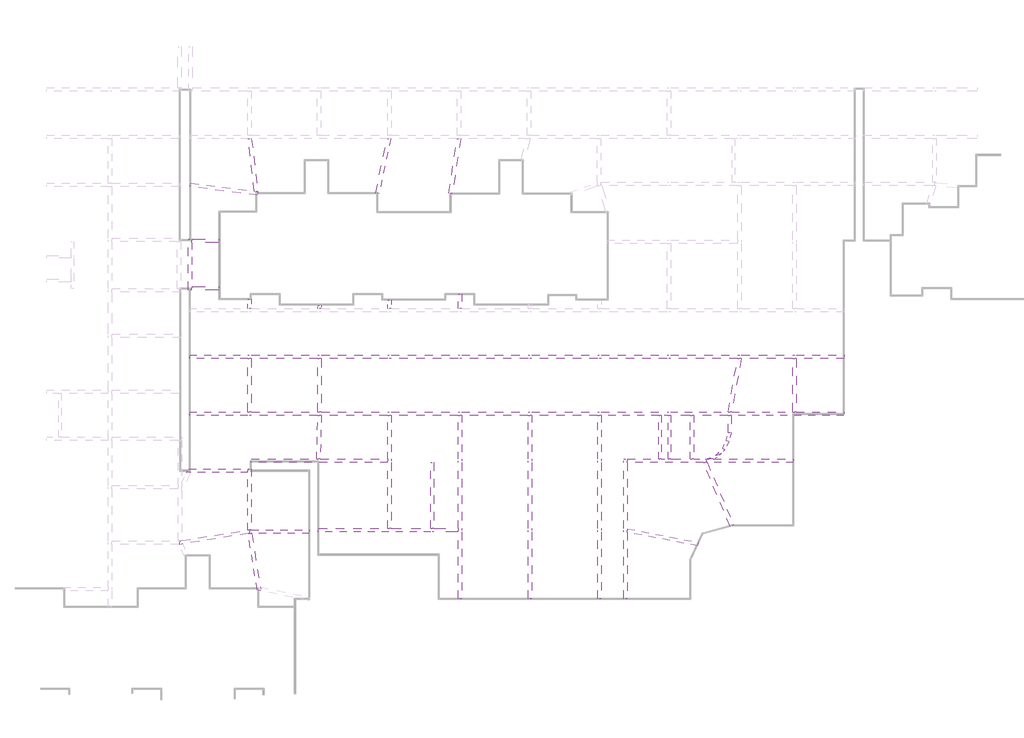
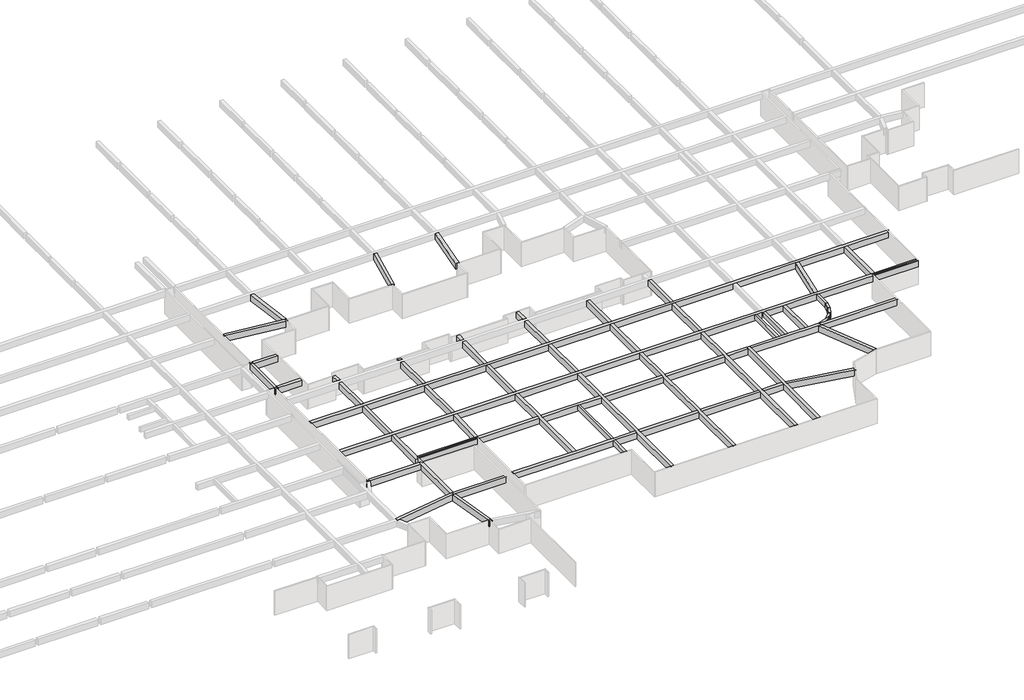
# One storey, part 12 of 16: 43 beams.
"""IFC4 building model written with IfcOpenShell, lengths in millimetres."""

from ifc_helpers import new_model, si_unit, frame, origin, place, context, project, spatial, polyline, outline, extrude, faceted_brep, element, save

model = new_model("IFC4")

# Units and contexts
model_context = context("Model", 3, world=origin())
ifc_project = project(units=[si_unit("LENGTHUNIT", "METRE", prefix="MILLI")], contexts=[model_context])

# Site, building, storey
site = spatial("IfcSite", under=ifc_project)
building = spatial("IfcBuilding", under=site)
storey = spatial("IfcBuildingStorey", under=building, Name="户型图", Elevation=0.0)

# Beams
placement = place(None, origin())
element("IfcBeam", 1, ObjectType="混凝土 - 矩形梁 : KL_beam", at=placement, inside=storey, context=model_context, shape_type="Brep", body=[
    faceted_brep([(256371.9419701, -178694.9170291, 3300.0), (255971.9419701, -178694.9170291, 3300.0), (255971.9419701, -184532.1273283, 3300.0), (256371.9419701, -184532.1273283, 3300.0), (256371.9419701, -184132.1273283, 3300.0), (256371.9419701, -179094.9170291, 3300.0), (256371.9419701, -178694.9170291, 2500.0), (256371.9419701, -184532.1273283, 2500.0), (256371.9419701, -184132.1273283, 2500.0), (256371.9419701, -179094.9170291, 2500.0), (255971.9419701, -178694.9170291, 2500.0), (255971.9419701, -184532.1273283, 2500.0)], [[[0, 1, 2, 3, 4, 5]], [[6, 0, 5, 4, 3, 7, 8, 9]], [[10, 6, 9, 8, 7, 11]], [[1, 10, 11, 2]], [[1, 0, 6, 10]], [[3, 2, 11, 7]]]),
])
element("IfcBeam", 2, ObjectType="混凝土 - 矩形梁 : KL_beam", at=placement, inside=storey, context=model_context, shape_type="Brep", body=[
    faceted_brep([(256229.1427512, -172325.6293063, 3300.0), (256229.1427512, -172325.6293063, 2500.0), (256178.5242086, -172722.4135842, 2500.0), (256178.5242086, -172722.4135842, 3300.0), (263858.3414133, -173702.1428111, 3300.0), (263908.9599559, -173305.3585333, 3300.0), (263499.8534109, -173253.1680152, 3300.0), (263858.3414133, -173702.1428111, 2500.0), (263908.9599559, -173305.3585333, 2500.0), (263499.8534109, -173253.1680152, 2500.0)], [[[0, 1, 2, 3]], [[4, 5, 6, 0, 3]], [[7, 4, 3, 2]], [[8, 7, 2, 1, 9]], [[5, 8, 9, 1, 0, 6]], [[5, 4, 7, 8]]]),
])
element("IfcBeam", 3, ObjectType="混凝土 - 矩形梁 : KL_beam", at=placement, inside=storey, context=model_context, shape_type="SweptSolid", body=[
    extrude(outline(polyline([(259423.0877072, -178694.9170291), (259423.0877072, -179094.9170291), (256371.9419701, -179094.9170291), (256371.9419701, -178694.9170291), (259423.0877072, -178694.9170291)])), frame((0.0, 0.0, 2500.0), z_axis=(0.0, 0.0, 1.0), x_axis=(1.0, 0.0, 0.0)), (0.0, 0.0, 1.0), 800.0),
])
element("IfcBeam", 4, ObjectType="混凝土 - 矩形梁 : KL_beam", at=placement, inside=storey, context=model_context, shape_type="SweptSolid", body=[
    extrude(outline(polyline([(259417.188018, -184132.1273283), (259417.188018, -184532.1273283), (256371.9419701, -184532.1273283), (256371.9419701, -184132.1273283), (259417.188018, -184132.1273283)])), frame((0.0, 0.0, 2500.0), z_axis=(0.0, 0.0, 1.0), x_axis=(1.0, 0.0, 0.0)), (0.0, 0.0, 1.0), 800.0),
])
element("IfcBeam", 5, ObjectType="混凝土 - 矩形梁 : KL_beam", at=placement, inside=storey, context=model_context, shape_type="Brep", body=[
    faceted_brep([(330953.597965, -191962.1668684, 3300.0), (330953.597965, -192362.1668684, 3300.0), (330953.597965, -192362.1668684, 2500.0), (330953.597965, -191962.1668684, 2500.0), (256118.597965, -191962.1668684, 3300.0), (256118.597965, -191962.1668684, 2500.0), (256118.597965, -192362.1668684, 2500.0), (256118.597965, -192362.1668684, 3300.0), (325452.9173169, -191962.1668684, 3300.0), (325052.9173169, -191962.1668684, 3300.0), (319175.2880408, -191962.1668684, 3300.0), (318775.2880408, -191962.1668684, 3300.0), (311075.2880408, -191962.1668684, 3300.0), (310675.2880408, -191962.1668684, 3300.0), (303155.2880408, -191962.1668684, 3300.0), (302755.2880408, -191962.1668684, 3300.0), (295188.9093069, -191962.1668684, 3300.0), (294788.9093069, -191962.1668684, 3300.0), (287188.9093069, -191962.1668684, 3300.0), (286788.9093069, -191962.1668684, 3300.0), (279139.4840766, -191962.1668684, 3300.0), (278739.4840766, -191962.1668684, 3300.0), (271154.6470805, -191962.1668684, 3300.0), (270754.6470805, -191962.1668684, 3300.0), (263153.757676, -191962.1668684, 3300.0), (262753.757676, -191962.1668684, 3300.0), (262753.757676, -192362.1668684, 3300.0), (263153.757676, -192362.1668684, 3300.0), (270754.6470805, -192362.1668684, 3300.0), (271154.6470805, -192362.1668684, 3300.0), (278739.4840766, -192362.1668684, 3300.0), (279139.4840766, -192362.1668684, 3300.0), (286788.9093069, -192362.1668684, 3300.0), (287188.9093069, -192362.1668684, 3300.0), (294788.9093069, -192362.1668684, 3300.0), (295188.9093069, -192362.1668684, 3300.0), (302755.2880408, -192362.1668684, 3300.0), (303155.2880408, -192362.1668684, 3300.0), (310675.2880408, -192362.1668684, 3300.0), (311075.2880408, -192362.1668684, 3300.0), (318737.3738799, -192362.1668684, 3300.0), (319143.4159061, -192362.1668684, 3300.0), (325052.9173169, -192362.1668684, 3300.0), (325452.9173169, -192362.1668684, 3300.0), (262753.757676, -192362.1668684, 2500.0), (263153.757676, -192362.1668684, 2500.0), (270754.6470805, -192362.1668684, 2500.0), (271154.6470805, -192362.1668684, 2500.0), (278739.4840766, -192362.1668684, 2500.0), (279139.4840766, -192362.1668684, 2500.0), (286788.9093069, -192362.1668684, 2500.0), (287188.9093069, -192362.1668684, 2500.0), (294788.9093069, -192362.1668684, 2500.0), (295188.9093069, -192362.1668684, 2500.0), (302755.2880408, -192362.1668684, 2500.0), (303155.2880408, -192362.1668684, 2500.0), (310675.2880408, -192362.1668684, 2500.0), (311075.2880408, -192362.1668684, 2500.0), (318737.3738799, -192362.1668684, 2500.0), (319143.4159061, -192362.1668684, 2500.0), (325052.9173169, -192362.1668684, 2500.0), (325452.9173169, -192362.1668684, 2500.0), (262753.757676, -191962.1668684, 2500.0), (263153.757676, -191962.1668684, 2500.0), (270754.6470805, -191962.1668684, 2500.0), (271154.6470805, -191962.1668684, 2500.0), (278739.4840766, -191962.1668684, 2500.0), (279139.4840766, -191962.1668684, 2500.0), (286788.9093069, -191962.1668684, 2500.0), (287188.9093069, -191962.1668684, 2500.0), (294788.9093069, -191962.1668684, 2500.0), (295188.9093069, -191962.1668684, 2500.0), (302755.2880408, -191962.1668684, 2500.0), (303155.2880408, -191962.1668684, 2500.0), (310675.2880408, -191962.1668684, 2500.0), (311075.2880408, -191962.1668684, 2500.0), (318775.2880408, -191962.1668684, 2500.0), (319175.2880408, -191962.1668684, 2500.0), (325052.9173169, -191962.1668684, 2500.0), (325452.9173169, -191962.1668684, 2500.0)], [[[0, 1, 2, 3]], [[4, 5, 6, 7]], [[1, 0, 8, 9, 10, 11, 12, 13, 14, 15, 16, 17, 18, 19, 20, 21, 22, 23, 24, 25, 4, 7, 26, 27, 28, 29, 30, 31, 32, 33, 34, 35, 36, 37, 38, 39, 40, 41, 42, 43]], [[2, 1, 43, 42, 41, 40, 39, 38, 37, 36, 35, 34, 33, 32, 31, 30, 29, 28, 27, 26, 7, 6, 44, 45, 46, 47, 48, 49, 50, 51, 52, 53, 54, 55, 56, 57, 58, 59, 60, 61]], [[3, 2, 61, 60, 59, 58, 57, 56, 55, 54, 53, 52, 51, 50, 49, 48, 47, 46, 45, 44, 6, 5, 62, 63, 64, 65, 66, 67, 68, 69, 70, 71, 72, 73, 74, 75, 76, 77, 78, 79]], [[0, 3, 79, 78, 77, 76, 75, 74, 73, 72, 71, 70, 69, 68, 67, 66, 65, 64, 63, 62, 5, 4, 25, 24, 23, 22, 21, 20, 19, 18, 17, 16, 15, 14, 13, 12, 11, 10, 9, 8]]]),
])
element("IfcBeam", 6, ObjectType="混凝土 - 矩形梁 : KL_beam", at=placement, inside=storey, context=model_context, shape_type="Brep", body=[
    faceted_brep([(330853.597965, -198470.1471774, 3300.0), (330853.597965, -198870.1471774, 3300.0), (330853.597965, -198870.1471774, 2500.0), (330853.597965, -198470.1471774, 2500.0), (256118.597965, -198470.1471774, 3300.0), (256118.597965, -198470.1471774, 2500.0), (256118.597965, -198870.1471774, 2500.0), (256118.597965, -198870.1471774, 3300.0), (325452.9173169, -198470.1471774, 3300.0), (325052.9173169, -198470.1471774, 3300.0), (318077.7826069, -198470.1471774, 3300.0), (317671.7405807, -198470.1471774, 3300.0), (311075.2880408, -198470.1471774, 3300.0), (310675.2880408, -198470.1471774, 3300.0), (303155.2880408, -198470.1471774, 3300.0), (302755.2880408, -198470.1471774, 3300.0), (295188.9093069, -198470.1471774, 3300.0), (294788.9093069, -198470.1471774, 3300.0), (287188.9093069, -198470.1471774, 3300.0), (286788.9093069, -198470.1471774, 3300.0), (279139.4840766, -198470.1471774, 3300.0), (278739.4840766, -198470.1471774, 3300.0), (271154.6470805, -198470.1471774, 3300.0), (270754.6470805, -198470.1471774, 3300.0), (263153.757676, -198470.1471774, 3300.0), (262753.757676, -198470.1471774, 3300.0), (262753.757676, -198870.1471774, 3300.0), (263153.757676, -198870.1471774, 3300.0), (270749.982593, -198870.1471774, 3300.0), (271150.0889009, -198870.1471774, 3300.0), (278739.4840766, -198870.1471774, 3300.0), (279139.4840766, -198870.1471774, 3300.0), (286788.9093069, -198870.1471774, 3300.0), (287188.9093069, -198870.1471774, 3300.0), (294788.9093069, -198870.1471774, 3300.0), (295188.9093069, -198870.1471774, 3300.0), (302755.2880408, -198870.1471774, 3300.0), (303155.2880408, -198870.1471774, 3300.0), (309705.2880408, -198870.1471774, 3300.0), (310005.2880408, -198870.1471774, 3300.0), (310675.2880408, -198870.1471774, 3300.0), (310805.2880408, -198870.1471774, 3300.0), (311105.2880408, -198870.1471774, 3300.0), (313355.2880408, -198870.1471774, 3300.0), (313755.2880408, -198870.1471774, 3300.0), (317689.868446, -198870.1471774, 3300.0), (317989.868446, -198870.1471774, 3300.0), (262753.757676, -198870.1471774, 2500.0), (263153.757676, -198870.1471774, 2500.0), (270749.982593, -198870.1471774, 2500.0), (271150.0889009, -198870.1471774, 2500.0), (278739.4840766, -198870.1471774, 2500.0), (279139.4840766, -198870.1471774, 2500.0), (286788.9093069, -198870.1471774, 2500.0), (287188.9093069, -198870.1471774, 2500.0), (294788.9093069, -198870.1471774, 2500.0), (295188.9093069, -198870.1471774, 2500.0), (302755.2880408, -198870.1471774, 2500.0), (303155.2880408, -198870.1471774, 2500.0), (310675.2880408, -198870.1471774, 2500.0), (311075.2880408, -198870.1471774, 2500.0), (313355.2880408, -198870.1471774, 2500.0), (313755.2880408, -198870.1471774, 2500.0), (262753.757676, -198470.1471774, 2500.0), (263153.757676, -198470.1471774, 2500.0), (270754.6470805, -198470.1471774, 2500.0), (271154.6470805, -198470.1471774, 2500.0), (278739.4840766, -198470.1471774, 2500.0), (279139.4840766, -198470.1471774, 2500.0), (286788.9093069, -198470.1471774, 2500.0), (287188.9093069, -198470.1471774, 2500.0), (294788.9093069, -198470.1471774, 2500.0), (295188.9093069, -198470.1471774, 2500.0), (302755.2880408, -198470.1471774, 2500.0), (303155.2880408, -198470.1471774, 2500.0), (310675.2880408, -198470.1471774, 2500.0), (311075.2880408, -198470.1471774, 2500.0), (317671.7405807, -198470.1471774, 2500.0), (318077.7826069, -198470.1471774, 2500.0), (325052.9173169, -198470.1471774, 2500.0), (325452.9173169, -198470.1471774, 2500.0)], [[[0, 1, 2, 3]], [[4, 5, 6, 7]], [[1, 0, 8, 9, 10, 11, 12, 13, 14, 15, 16, 17, 18, 19, 20, 21, 22, 23, 24, 25, 4, 7, 26, 27, 28, 29, 30, 31, 32, 33, 34, 35, 36, 37, 38, 39, 40, 41, 42, 43, 44, 45, 46]], [[2, 1, 46, 45, 44, 43, 42, 41, 40, 39, 38, 37, 36, 35, 34, 33, 32, 31, 30, 29, 28, 27, 26, 7, 6, 47, 48, 49, 50, 51, 52, 53, 54, 55, 56, 57, 58, 59, 60, 61, 62]], [[3, 2, 62, 61, 60, 59, 58, 57, 56, 55, 54, 53, 52, 51, 50, 49, 48, 47, 6, 5, 63, 64, 65, 66, 67, 68, 69, 70, 71, 72, 73, 74, 75, 76, 77, 78, 79, 80]], [[0, 3, 80, 79, 78, 77, 76, 75, 74, 73, 72, 71, 70, 69, 68, 67, 66, 65, 64, 63, 5, 4, 25, 24, 23, 22, 21, 20, 19, 18, 17, 16, 15, 14, 13, 12, 11, 10, 9, 8]]]),
])
element("IfcBeam", 7, ObjectType="混凝土 - 矩形梁 : KL_beam", at=placement, inside=storey, context=model_context, shape_type="Brep", body=[
    faceted_brep([(262753.757676, -204304.6570229, 3300.0), (262753.757676, -204304.6570229, 2500.0), (263153.757676, -204304.6570229, 2500.0), (263153.757676, -204304.6570229, 3300.0), (262753.757676, -198870.1471774, 3300.0), (263153.757676, -198870.1471774, 3300.0), (263153.757676, -198870.1471774, 2500.0), (262753.757676, -198870.1471774, 2500.0), (263153.757676, -204273.7545432, 3300.0), (263153.757676, -203873.7545432, 3300.0), (263153.757676, -204273.7545432, 2500.0), (263153.757676, -203873.7545432, 2500.0)], [[[0, 1, 2, 3]], [[4, 5, 6, 7]], [[0, 3, 8, 9, 5, 4]], [[3, 2, 10, 11, 6, 5, 9, 8]], [[2, 1, 7, 6, 11, 10]], [[1, 0, 4, 7]]]),
    faceted_brep([(263153.757676, -187062.1668684, 3300.0), (262753.757676, -187062.1668684, 3300.0), (262753.757676, -191962.1668684, 3300.0), (263153.757676, -191962.1668684, 3300.0), (263153.757676, -187062.1668684, 2500.0), (263153.757676, -191962.1668684, 2500.0), (262753.757676, -187062.1668684, 2500.0), (262753.757676, -191962.1668684, 2500.0)], [[[0, 1, 2, 3]], [[4, 0, 3, 5]], [[6, 4, 5, 7]], [[1, 6, 7, 2]], [[1, 0, 4, 6]], [[3, 2, 7, 5]]]),
    faceted_brep([(262753.757676, -192362.1668684, 3300.0), (263153.757676, -192362.1668684, 3300.0), (263153.757676, -192362.1668684, 2500.0), (262753.757676, -192362.1668684, 2500.0), (262753.757676, -198470.1471774, 3300.0), (263153.757676, -198470.1471774, 3300.0), (263153.757676, -198470.1471774, 2500.0), (262753.757676, -198470.1471774, 2500.0)], [[[0, 1, 2, 3]], [[1, 0, 4, 5]], [[2, 1, 5, 6]], [[3, 2, 6, 7]], [[0, 3, 7, 4]], [[5, 4, 7, 6]]]),
])
element("IfcBeam", 8, ObjectType="混凝土 - 矩形梁 : KL_beam", at=placement, inside=storey, context=model_context, shape_type="SweptSolid", body=[
    extrude(outline(polyline([(270754.6470805, -187062.1668684), (271154.6470805, -187062.1668684), (271154.6470805, -191962.1668684), (270754.6470805, -191962.1668684), (270754.6470805, -187062.1668684)])), frame((0.0, 0.0, 2500.0), z_axis=(0.0, 0.0, 1.0), x_axis=(1.0, 0.0, 0.0)), (0.0, 0.0, 1.0), 800.0),
    extrude(outline(polyline([(271154.6470805, -198470.1471774), (270754.6470805, -198470.1471774), (270754.6470805, -192362.1668684), (271154.6470805, -192362.1668684), (271154.6470805, -198470.1471774)])), frame((0.0, 0.0, 2500.0), z_axis=(0.0, 0.0, 1.0), x_axis=(1.0, 0.0, 0.0)), (0.0, 0.0, 1.0), 800.0),
])
element("IfcBeam", 9, ObjectType="混凝土 - 矩形梁 : KL_beam", at=placement, inside=storey, context=model_context, shape_type="SweptSolid", body=[
    extrude(outline(polyline([(270749.982593, -198870.1471774), (271150.0889009, -198870.1471774), (271034.7223897, -203873.7545432), (270634.6160818, -203873.7545432), (270749.982593, -198870.1471774)])), frame((0.0, 0.0, 2500.0), z_axis=(0.0, 0.0, 1.0), x_axis=(1.0, 0.0, 0.0)), (0.0, 0.0, 1.0), 800.0),
])
element("IfcBeam", 10, ObjectType="混凝土 - 矩形梁 : KL_beam", at=placement, inside=storey, context=model_context, shape_type="Brep", body=[
    faceted_brep([(279139.4840766, -198870.1471774, 3300.0), (278739.4840766, -198870.1471774, 3300.0), (278739.4840766, -203873.7545432, 3300.0), (278739.4840766, -204273.7545432, 3300.0), (278739.4840766, -211805.8350287, 3300.0), (279139.4840766, -211805.8350287, 3300.0), (279139.4840766, -204273.7545432, 3300.0), (279139.4840766, -203873.7545432, 3300.0), (279139.4840766, -198870.1471774, 2500.0), (279139.4840766, -211805.8350287, 2500.0), (279139.4840766, -204273.7545432, 2500.0), (279139.4840766, -203873.7545432, 2500.0), (278739.4840766, -198870.1471774, 2500.0), (278739.4840766, -211805.8350287, 2500.0), (278739.4840766, -204273.7545432, 2500.0), (278739.4840766, -203873.7545432, 2500.0)], [[[0, 1, 2, 3, 4, 5, 6, 7]], [[8, 0, 7, 6, 5, 9, 10, 11]], [[12, 8, 11, 10, 9, 13, 14, 15]], [[1, 12, 15, 14, 13, 4, 3, 2]], [[1, 0, 8, 12]], [[5, 4, 13, 9]]]),
    faceted_brep([(278739.4840766, -187062.1668684, 3300.0), (279139.4840766, -187062.1668684, 3300.0), (279139.4840766, -187062.1668684, 2500.0), (278739.4840766, -187062.1668684, 2500.0), (279139.4840766, -191962.1668684, 3300.0), (278739.4840766, -191962.1668684, 3300.0), (278739.4840766, -191962.1668684, 2500.0), (279139.4840766, -191962.1668684, 2500.0)], [[[0, 1, 2, 3]], [[4, 5, 6, 7]], [[1, 0, 5, 4]], [[2, 1, 4, 7]], [[3, 2, 7, 6]], [[0, 3, 6, 5]]]),
    faceted_brep([(278739.4840766, -192362.1668684, 3300.0), (279139.4840766, -192362.1668684, 3300.0), (279139.4840766, -192362.1668684, 2500.0), (278739.4840766, -192362.1668684, 2500.0), (279139.4840766, -198470.1471774, 3300.0), (278739.4840766, -198470.1471774, 3300.0), (278739.4840766, -198470.1471774, 2500.0), (279139.4840766, -198470.1471774, 2500.0)], [[[0, 1, 2, 3]], [[4, 5, 6, 7]], [[1, 0, 5, 4]], [[2, 1, 4, 7]], [[3, 2, 7, 6]], [[0, 3, 6, 5]]]),
])
element("IfcBeam", 11, ObjectType="混凝土 - 矩形梁 : KL_beam", at=placement, inside=storey, context=model_context, shape_type="Brep", body=[
    faceted_brep([(287188.9093069, -219873.4607058, 3300.0), (286788.9093069, -219873.4607058, 3300.0), (286788.9093069, -219873.4607058, 2500.0), (287188.9093069, -219873.4607058, 2500.0), (287188.9093069, -212205.8350287, 3300.0), (287188.9093069, -211805.8350287, 3300.0), (287188.9093069, -204273.7545432, 3300.0), (287188.9093069, -203873.7545432, 3300.0), (287188.9093069, -198870.1471774, 3300.0), (286788.9093069, -198870.1471774, 3300.0), (286788.9093069, -203873.7545432, 3300.0), (286788.9093069, -204273.7545432, 3300.0), (286788.9093069, -211805.8350287, 3300.0), (286788.9093069, -212205.8350287, 3300.0), (286788.9093069, -198870.1471774, 2500.0), (286788.9093069, -203873.7545432, 2500.0), (286788.9093069, -204273.7545432, 2500.0), (286788.9093069, -211805.8350287, 2500.0), (286788.9093069, -212205.8350287, 2500.0), (287188.9093069, -198870.1471774, 2500.0), (287188.9093069, -203873.7545432, 2500.0), (287188.9093069, -204273.7545432, 2500.0), (287188.9093069, -211805.8350287, 2500.0), (287188.9093069, -212205.8350287, 2500.0)], [[[0, 1, 2, 3]], [[1, 0, 4, 5, 6, 7, 8, 9, 10, 11, 12, 13]], [[2, 1, 13, 12, 11, 10, 9, 14, 15, 16, 17, 18]], [[3, 2, 18, 17, 16, 15, 14, 19, 20, 21, 22, 23]], [[0, 3, 23, 22, 21, 20, 19, 8, 7, 6, 5, 4]], [[9, 8, 19, 14]]]),
    faceted_brep([(286788.9093069, -187062.1668684, 3300.0), (287188.9093069, -187062.1668684, 3300.0), (287188.9093069, -187062.1668684, 2500.0), (286788.9093069, -187062.1668684, 2500.0), (287188.9093069, -191962.1668684, 3300.0), (286788.9093069, -191962.1668684, 3300.0), (286788.9093069, -191962.1668684, 2500.0), (287188.9093069, -191962.1668684, 2500.0)], [[[0, 1, 2, 3]], [[4, 5, 6, 7]], [[1, 0, 5, 4]], [[0, 3, 6, 5]], [[3, 2, 7, 6]], [[2, 1, 4, 7]]]),
    faceted_brep([(286788.9093069, -192362.1668684, 3300.0), (287188.9093069, -192362.1668684, 3300.0), (287188.9093069, -192362.1668684, 2500.0), (286788.9093069, -192362.1668684, 2500.0), (287188.9093069, -198470.1471774, 3300.0), (286788.9093069, -198470.1471774, 3300.0), (286788.9093069, -198470.1471774, 2500.0), (287188.9093069, -198470.1471774, 2500.0)], [[[0, 1, 2, 3]], [[4, 5, 6, 7]], [[1, 0, 5, 4]], [[0, 3, 6, 5]], [[3, 2, 7, 6]], [[2, 1, 4, 7]]]),
])
element("IfcBeam", 12, ObjectType="混凝土 - 矩形梁 : KL_beam", at=placement, inside=storey, context=model_context, shape_type="Brep", body=[
    faceted_brep([(294788.9093069, -219873.4607058, 3300.0), (294788.9093069, -219873.4607058, 2500.0), (295188.9093069, -219873.4607058, 2500.0), (295188.9093069, -219873.4607058, 3300.0), (294788.9093069, -198870.1471774, 3300.0), (295188.9093069, -198870.1471774, 3300.0), (295188.9093069, -198870.1471774, 2500.0), (294788.9093069, -198870.1471774, 2500.0), (295188.9093069, -212205.8350287, 3300.0), (295188.9093069, -211805.8350287, 3300.0), (295188.9093069, -204273.7545432, 3300.0), (295188.9093069, -203873.7545432, 3300.0), (294788.9093069, -203873.7545432, 3300.0), (294788.9093069, -204273.7545432, 3300.0), (294788.9093069, -211805.8350287, 3300.0), (294788.9093069, -212205.8350287, 3300.0), (295188.9093069, -212205.8350287, 2500.0), (295188.9093069, -211805.8350287, 2500.0), (295188.9093069, -204273.7545432, 2500.0), (295188.9093069, -203873.7545432, 2500.0), (294788.9093069, -212205.8350287, 2500.0), (294788.9093069, -211805.8350287, 2500.0), (294788.9093069, -204273.7545432, 2500.0), (294788.9093069, -203873.7545432, 2500.0)], [[[0, 1, 2, 3]], [[4, 5, 6, 7]], [[0, 3, 8, 9, 10, 11, 5, 4, 12, 13, 14, 15]], [[3, 2, 16, 17, 18, 19, 6, 5, 11, 10, 9, 8]], [[2, 1, 20, 21, 22, 23, 7, 6, 19, 18, 17, 16]], [[1, 0, 15, 14, 13, 12, 4, 7, 23, 22, 21, 20]]]),
    faceted_brep([(295188.9093069, -187062.1668684, 3300.0), (294788.9093069, -187062.1668684, 3300.0), (294788.9093069, -191962.1668684, 3300.0), (295188.9093069, -191962.1668684, 3300.0), (295188.9093069, -187062.1668684, 2500.0), (295188.9093069, -191962.1668684, 2500.0), (294788.9093069, -187062.1668684, 2500.0), (294788.9093069, -191962.1668684, 2500.0)], [[[0, 1, 2, 3]], [[4, 0, 3, 5]], [[6, 4, 5, 7]], [[1, 6, 7, 2]], [[1, 0, 4, 6]], [[3, 2, 7, 5]]]),
    faceted_brep([(294788.9093069, -192362.1668684, 3300.0), (295188.9093069, -192362.1668684, 3300.0), (295188.9093069, -192362.1668684, 2500.0), (294788.9093069, -192362.1668684, 2500.0), (294788.9093069, -198470.1471774, 3300.0), (295188.9093069, -198470.1471774, 3300.0), (295188.9093069, -198470.1471774, 2500.0), (294788.9093069, -198470.1471774, 2500.0)], [[[0, 1, 2, 3]], [[1, 0, 4, 5]], [[2, 1, 5, 6]], [[3, 2, 6, 7]], [[0, 3, 7, 4]], [[5, 4, 7, 6]]]),
])
element("IfcBeam", 13, ObjectType="混凝土 - 矩形梁 : KL_beam", at=placement, inside=storey, context=model_context, shape_type="Brep", body=[
    faceted_brep([(303155.2880408, -219873.4607058, 3300.0), (302755.2880408, -219873.4607058, 3300.0), (302755.2880408, -219873.4607058, 2500.0), (303155.2880408, -219873.4607058, 2500.0), (303155.2880408, -212205.8350287, 3300.0), (303155.2880408, -211805.8350287, 3300.0), (303155.2880408, -204273.7545432, 3300.0), (303155.2880408, -203873.7545432, 3300.0), (303155.2880408, -198870.1471774, 3300.0), (302755.2880408, -198870.1471774, 3300.0), (302755.2880408, -203873.7545432, 3300.0), (302755.2880408, -204273.7545432, 3300.0), (302755.2880408, -211805.8350287, 3300.0), (302755.2880408, -212205.8350287, 3300.0), (302755.2880408, -198870.1471774, 2500.0), (302755.2880408, -203873.7545432, 2500.0), (302755.2880408, -204273.7545432, 2500.0), (302755.2880408, -211805.8350287, 2500.0), (302755.2880408, -212205.8350287, 2500.0), (303155.2880408, -198870.1471774, 2500.0), (303155.2880408, -203873.7545432, 2500.0), (303155.2880408, -204273.7545432, 2500.0), (303155.2880408, -211805.8350287, 2500.0), (303155.2880408, -212205.8350287, 2500.0)], [[[0, 1, 2, 3]], [[1, 0, 4, 5, 6, 7, 8, 9, 10, 11, 12, 13]], [[2, 1, 13, 12, 11, 10, 9, 14, 15, 16, 17, 18]], [[3, 2, 18, 17, 16, 15, 14, 19, 20, 21, 22, 23]], [[0, 3, 23, 22, 21, 20, 19, 8, 7, 6, 5, 4]], [[9, 8, 19, 14]]]),
    faceted_brep([(302755.2880408, -187062.1668684, 3300.0), (303155.2880408, -187062.1668684, 3300.0), (303155.2880408, -187062.1668684, 2500.0), (302755.2880408, -187062.1668684, 2500.0), (303155.2880408, -191962.1668684, 3300.0), (302755.2880408, -191962.1668684, 3300.0), (302755.2880408, -191962.1668684, 2500.0), (303155.2880408, -191962.1668684, 2500.0)], [[[0, 1, 2, 3]], [[4, 5, 6, 7]], [[1, 0, 5, 4]], [[0, 3, 6, 5]], [[3, 2, 7, 6]], [[2, 1, 4, 7]]]),
    faceted_brep([(302755.2880408, -192362.1668684, 3300.0), (303155.2880408, -192362.1668684, 3300.0), (303155.2880408, -192362.1668684, 2500.0), (302755.2880408, -192362.1668684, 2500.0), (303155.2880408, -198470.1471774, 3300.0), (302755.2880408, -198470.1471774, 3300.0), (302755.2880408, -198470.1471774, 2500.0), (303155.2880408, -198470.1471774, 2500.0)], [[[0, 1, 2, 3]], [[4, 5, 6, 7]], [[1, 0, 5, 4]], [[0, 3, 6, 5]], [[3, 2, 7, 6]], [[2, 1, 4, 7]]]),
])
element("IfcBeam", 14, ObjectType="混凝土 - 矩形梁 : KL_beam", at=placement, inside=storey, context=model_context, shape_type="Brep", body=[
    faceted_brep([(305755.2880408, -219873.7545432, 3300.0), (305755.2880408, -219873.7545432, 2500.0), (306155.2880408, -219873.7545432, 2500.0), (306155.2880408, -219873.7545432, 3300.0), (306155.2880408, -212248.4544295, 3300.0), (306155.2880408, -211840.9677515, 3300.0), (306155.2880408, -204273.7545432, 3300.0), (306155.2880408, -203873.7545432, 3300.0), (305755.2880408, -203873.7545432, 3300.0), (305755.2880408, -204273.7545432, 3300.0), (305755.2880408, -211805.8350287, 3300.0), (305755.2880408, -212205.8350287, 3300.0), (306155.2880408, -212248.4544295, 2500.0), (306155.2880408, -211840.9677515, 2500.0), (306155.2880408, -204273.7545432, 2500.0), (306155.2880408, -203873.7545432, 2500.0), (305755.2880408, -212205.8350287, 2500.0), (305755.2880408, -211805.8350287, 2500.0), (305755.2880408, -204273.7545432, 2500.0), (305755.2880408, -203873.7545432, 2500.0)], [[[0, 1, 2, 3]], [[0, 3, 4, 5, 6, 7, 8, 9, 10, 11]], [[3, 2, 12, 13, 14, 15, 7, 6, 5, 4]], [[2, 1, 16, 17, 18, 19, 15, 14, 13, 12]], [[1, 0, 11, 10, 9, 8, 19, 18, 17, 16]], [[8, 7, 15, 19]]]),
])
element("IfcBeam", 15, ObjectType="混凝土 - 矩形梁 : KL_beam", at=placement, inside=storey, context=model_context, shape_type="Brep", body=[
    faceted_brep([(315257.2223737, -204273.7545432, 3300.0), (315087.7671783, -203873.7545432, 3300.0), (315066.2128647, -203873.7545432, 3300.0), (313755.2880408, -203873.7545432, 3300.0), (313355.2880408, -203873.7545432, 3300.0), (311105.2880408, -203873.7545432, 3300.0), (310805.2880408, -203873.7545432, 3300.0), (310005.2880408, -203873.7545432, 3300.0), (309705.2880408, -203873.7545432, 3300.0), (306155.2880408, -203873.7545432, 3300.0), (306155.2880408, -204273.7545432, 3300.0), (314822.8089033, -204273.7545432, 3300.0), (315257.2223737, -204273.7545432, 2500.0), (306155.2880408, -204273.7545432, 2500.0), (314822.8089033, -204273.7545432, 2500.0), (315087.7671783, -203873.7545432, 2500.0), (306155.2880408, -203873.7545432, 2500.0), (313355.2880408, -203873.7545432, 2500.0), (313755.2880408, -203873.7545432, 2500.0)], [[[0, 1, 2, 3, 4, 5, 6, 7, 8, 9, 10, 11]], [[12, 0, 11, 10, 13, 14]], [[15, 12, 14, 13, 16, 17, 18]], [[1, 15, 18, 17, 16, 9, 8, 7, 6, 5, 4, 3, 2]], [[10, 9, 16, 13]], [[1, 0, 12, 15]]]),
])
element("IfcBeam", 16, ObjectType="混凝土 - 矩形梁 : KL_beam", at=placement, inside=storey, context=model_context, shape_type="Brep", body=[
    faceted_brep([(325092.6026789, -203873.7545432, 3300.0), (325092.6026789, -204273.7545432, 3300.0), (325092.6026789, -204273.7545432, 2500.0), (325092.6026789, -203873.7545432, 2500.0), (315943.3541847, -203873.7545432, 3300.0), (315087.7671783, -203873.7545432, 3300.0), (315257.2223737, -204273.7545432, 3300.0), (315257.2223737, -204273.7545432, 2500.0), (315087.7671783, -203873.7545432, 2500.0)], [[[0, 1, 2, 3]], [[1, 0, 4, 5, 6]], [[2, 1, 6, 7]], [[3, 2, 7, 8]], [[0, 3, 8, 5, 4]], [[6, 5, 8, 7]]]),
])
element("IfcBeam", 17, ObjectType="混凝土 - 矩形梁 : KL_beam", at=placement, inside=storey, context=model_context, shape_type="SweptSolid", body=[
    extrude(outline(polyline([(313355.2880408, -198870.1471774), (313755.2880408, -198870.1471774), (313755.2880408, -203873.7545432), (313355.2880408, -203873.7545432), (313355.2880408, -198870.1471774)])), frame((0.0, 0.0, 2500.0), z_axis=(0.0, 0.0, 1.0), x_axis=(1.0, 0.0, 0.0)), (0.0, 0.0, 1.0), 800.0),
])
element("IfcBeam", 18, ObjectType="混凝土 - 矩形梁 : KL_beam", at=placement, inside=storey, context=model_context, shape_type="Brep", body=[
    faceted_brep([(305755.2880408, -204273.7545432, 3300.0), (305755.2880408, -203873.7545432, 3300.0), (303155.2880408, -203873.7545432, 3300.0), (303155.2880408, -204273.7545432, 3300.0), (305755.2880408, -203873.7545432, 2500.0), (303155.2880408, -203873.7545432, 2500.0), (305755.2880408, -204273.7545432, 2500.0), (303155.2880408, -204273.7545432, 2500.0)], [[[0, 1, 2, 3]], [[1, 4, 5, 2]], [[4, 6, 7, 5]], [[6, 0, 3, 7]], [[1, 0, 6, 4]], [[3, 2, 5, 7]]]),
    faceted_brep([(263153.757676, -204273.7545432, 3300.0), (263153.757676, -203873.7545432, 3300.0), (263153.757676, -203873.7545432, 2500.0), (263153.757676, -204273.7545432, 2500.0), (278739.4840766, -203873.7545432, 3300.0), (278739.4840766, -204273.7545432, 3300.0), (278739.4840766, -204273.7545432, 2500.0), (278739.4840766, -203873.7545432, 2500.0), (271034.7223897, -203873.7545432, 3300.0), (270634.6160818, -203873.7545432, 3300.0), (271034.7223897, -203873.7545432, 2500.0), (270634.6160818, -203873.7545432, 2500.0)], [[[0, 1, 2, 3]], [[4, 5, 6, 7]], [[1, 0, 5, 4, 8, 9]], [[2, 1, 9, 8, 4, 7, 10, 11]], [[3, 2, 11, 10, 7, 6]], [[0, 3, 6, 5]]]),
    faceted_brep([(279139.4840766, -204273.7545432, 3300.0), (279139.4840766, -203873.7545432, 3300.0), (279139.4840766, -203873.7545432, 2500.0), (279139.4840766, -204273.7545432, 2500.0), (286788.9093069, -203873.7545432, 3300.0), (286788.9093069, -204273.7545432, 3300.0), (286788.9093069, -204273.7545432, 2500.0), (286788.9093069, -203873.7545432, 2500.0), (283693.7576761, -204273.7545432, 3300.0), (283993.7576761, -204273.7545432, 3300.0)], [[[0, 1, 2, 3]], [[4, 5, 6, 7]], [[1, 0, 8, 9, 5, 4]], [[2, 1, 4, 7]], [[3, 2, 7, 6]], [[0, 3, 6, 5, 9, 8]]]),
    faceted_brep([(287188.9093069, -204273.7545432, 3300.0), (287188.9093069, -203873.7545432, 3300.0), (287188.9093069, -203873.7545432, 2500.0), (287188.9093069, -204273.7545432, 2500.0), (294788.9093069, -203873.7545432, 3300.0), (294788.9093069, -204273.7545432, 3300.0), (294788.9093069, -204273.7545432, 2500.0), (294788.9093069, -203873.7545432, 2500.0)], [[[0, 1, 2, 3]], [[4, 5, 6, 7]], [[1, 0, 5, 4]], [[2, 1, 4, 7]], [[3, 2, 7, 6]], [[0, 3, 6, 5]]]),
    faceted_brep([(295188.9093069, -204273.7545432, 3300.0), (295188.9093069, -203873.7545432, 3300.0), (295188.9093069, -203873.7545432, 2500.0), (295188.9093069, -204273.7545432, 2500.0), (302755.2880408, -203873.7545432, 3300.0), (302755.2880408, -204273.7545432, 3300.0), (302755.2880408, -204273.7545432, 2500.0), (302755.2880408, -203873.7545432, 2500.0)], [[[0, 1, 2, 3]], [[4, 5, 6, 7]], [[1, 0, 5, 4]], [[2, 1, 4, 7]], [[3, 2, 7, 6]], [[0, 3, 6, 5]]]),
])
element("IfcBeam", 19, ObjectType="混凝土 - 矩形梁 : KL_beam", at=placement, inside=storey, context=model_context, shape_type="Brep", body=[
    faceted_brep([(270829.0228584, -211805.8350287, 3300.0), (270829.0228584, -211805.8350287, 2500.0), (270829.0228584, -212205.8350287, 2500.0), (270829.0228584, -212205.8350287, 3300.0), (286788.9093069, -211805.8350287, 3300.0), (286788.9093069, -212205.8350287, 3300.0), (286788.9093069, -212205.8350287, 2500.0), (286788.9093069, -211805.8350287, 2500.0), (283693.7576761, -212205.8350287, 3300.0), (283993.7576761, -212205.8350287, 3300.0), (283993.7576761, -211805.8350287, 3300.0), (283693.7576761, -211805.8350287, 3300.0), (279139.4840766, -211805.8350287, 3300.0), (278739.4840766, -211805.8350287, 3300.0), (278739.4840766, -211805.8350287, 2500.0), (279139.4840766, -211805.8350287, 2500.0)], [[[0, 1, 2, 3]], [[4, 5, 6, 7]], [[0, 3, 8, 9, 5, 4, 10, 11, 12, 13]], [[3, 2, 6, 5, 9, 8]], [[2, 1, 14, 15, 7, 6]], [[1, 0, 13, 12, 11, 10, 4, 7, 15, 14]]]),
    faceted_brep([(287188.9093069, -211805.8350287, 3300.0), (287188.9093069, -212205.8350287, 3300.0), (294788.9093069, -212205.8350287, 3300.0), (294788.9093069, -211805.8350287, 3300.0), (287188.9093069, -212205.8350287, 2500.0), (294788.9093069, -212205.8350287, 2500.0), (287188.9093069, -211805.8350287, 2500.0), (294788.9093069, -211805.8350287, 2500.0)], [[[0, 1, 2, 3]], [[1, 4, 5, 2]], [[4, 6, 7, 5]], [[6, 0, 3, 7]], [[1, 0, 6, 4]], [[3, 2, 5, 7]]]),
    faceted_brep([(305755.2880408, -211805.8350287, 3300.0), (305755.2880408, -212205.8350287, 3300.0), (305755.2880408, -212205.8350287, 2500.0), (305755.2880408, -211805.8350287, 2500.0), (303155.2880408, -211805.8350287, 3300.0), (303155.2880408, -212205.8350287, 3300.0), (303155.2880408, -212205.8350287, 2500.0), (303155.2880408, -211805.8350287, 2500.0)], [[[0, 1, 2, 3]], [[1, 0, 4, 5]], [[2, 1, 5, 6]], [[3, 2, 6, 7]], [[0, 3, 7, 4]], [[5, 4, 7, 6]]]),
    faceted_brep([(295188.9093069, -212205.8350287, 3300.0), (295188.9093069, -211805.8350287, 3300.0), (295188.9093069, -211805.8350287, 2500.0), (295188.9093069, -212205.8350287, 2500.0), (302755.2880408, -211805.8350287, 3300.0), (302755.2880408, -212205.8350287, 3300.0), (302755.2880408, -212205.8350287, 2500.0), (302755.2880408, -211805.8350287, 2500.0)], [[[0, 1, 2, 3]], [[4, 5, 6, 7]], [[1, 0, 5, 4]], [[0, 3, 6, 5]], [[3, 2, 7, 6]], [[2, 1, 4, 7]]]),
])
element("IfcBeam", 20, ObjectType="混凝土 - 矩形梁 : KL_beam", at=placement, inside=storey, context=model_context, shape_type="SweptSolid", body=[
    extrude(outline(polyline([(314239.1181809, -213412.3051532), (314162.7945827, -213804.9560265), (306155.2880408, -212248.4544295), (306155.2880408, -211840.9677515), (314239.1181809, -213412.3051532)])), frame((0.0, 0.0, 2500.0), z_axis=(0.0, 0.0, 1.0), x_axis=(1.0, 0.0, 0.0)), (0.0, 0.0, 1.0), 800.0),
])
element("IfcBeam", 21, ObjectType="混凝土 - 矩形梁 : KL_beam", at=placement, inside=storey, context=model_context, shape_type="SweptSolid", body=[
    extrude(outline(polyline([(318276.9582415, -211401.8590835), (317908.6455373, -211557.8903366), (314822.8089033, -204273.7545432), (315257.2223737, -204273.7545432), (318276.9582415, -211401.8590835)])), frame((0.0, 0.0, 2500.0), z_axis=(0.0, 0.0, 1.0), x_axis=(1.0, 0.0, 0.0)), (0.0, 0.0, 1.0), 800.0),
])
element("IfcBeam", 22, ObjectType="混凝土 - 矩形梁 : KL_beam", at=placement, inside=storey, context=model_context, shape_type="SweptSolid", body=[
    extrude(outline(polyline([(286788.9093069, -185002.1668684), (287188.9093069, -185002.1668684), (287188.9093069, -186662.1668684), (286788.9093069, -186662.1668684), (286788.9093069, -185002.1668684)])), frame((0.0, 0.0, 2500.0), z_axis=(0.0, 0.0, 1.0), x_axis=(1.0, 0.0, 0.0)), (0.0, 0.0, 1.0), 800.0),
])
element("IfcBeam", 23, ObjectType="混凝土 - 矩形梁 : KL_beam", at=placement, inside=storey, context=model_context, shape_type="SweptSolid", body=[
    extrude(outline(polyline([(278739.4840766, -185716.1541669), (279139.4840766, -185716.1541669), (279139.4840766, -186662.1668684), (278739.4840766, -186662.1668684), (278739.4840766, -185716.1541669)])), frame((0.0, 0.0, 2500.0), z_axis=(0.0, 0.0, 1.0), x_axis=(1.0, 0.0, 0.0)), (0.0, 0.0, 1.0), 800.0),
])
element("IfcBeam", 24, ObjectType="混凝土 - 矩形梁 : KL_beam", at=placement, inside=storey, context=model_context, shape_type="SweptSolid", body=[
    extrude(outline(polyline([(270754.6470805, -186307.6992344), (271154.6470805, -186307.6992344), (271154.6470805, -186662.1668684), (270754.6470805, -186662.1668684), (270754.6470805, -186307.6992344)])), frame((0.0, 0.0, 2500.0), z_axis=(0.0, 0.0, 1.0), x_axis=(1.0, 0.0, 0.0)), (0.0, 0.0, 1.0), 800.0),
])
element("IfcBeam", 25, ObjectType="混凝土 - 矩形梁 : KL_beam", at=placement, inside=storey, context=model_context, shape_type="SweptSolid", body=[
    extrude(outline(polyline([(262753.757676, -185584.0893216), (263153.757676, -185584.0893216), (263153.757676, -186662.1668684), (262753.757676, -186662.1668684), (262753.757676, -185584.0893216)])), frame((0.0, 0.0, 2500.0), z_axis=(0.0, 0.0, 1.0), x_axis=(1.0, 0.0, 0.0)), (0.0, 0.0, 1.0), 800.0),
])
element("IfcBeam", 26, ObjectType="混凝土 - 矩形梁 : KL_beam", at=placement, inside=storey, context=model_context, shape_type="SweptSolid", body=[
    extrude(outline(polyline([(263908.9599559, -173305.3585333), (263499.8534109, -173253.1680152), (262777.848794, -167223.3600959), (263180.706086, -167223.3600959), (263908.9599559, -173305.3585333)])), frame((0.0, 0.0, 2500.0), z_axis=(0.0, 0.0, 1.0), x_axis=(1.0, 0.0, 0.0)), (0.0, 0.0, 1.0), 800.0),
])
element("IfcBeam", 27, ObjectType="混凝土 - 矩形梁 : KL_beam", at=placement, inside=storey, context=model_context, shape_type="SweptSolid", body=[
    extrude(outline(polyline([(277762.1626855, -173525.1116511), (277370.9036452, -173441.9469748), (278692.7050906, -167223.3600959), (279101.6413286, -167223.3600959), (277762.1626855, -173525.1116511)])), frame((0.0, 0.0, 2500.0), z_axis=(0.0, 0.0, 1.0), x_axis=(1.0, 0.0, 0.0)), (0.0, 0.0, 1.0), 800.0),
])
element("IfcBeam", 28, ObjectType="混凝土 - 矩形梁 : KL_beam", at=placement, inside=storey, context=model_context, shape_type="SweptSolid", body=[
    extrude(outline(polyline([(286126.7736467, -173533.1654146), (285731.1875911, -173473.9060475), (286667.5284745, -167223.3600959), (287071.9916696, -167223.3600959), (286126.7736467, -173533.1654146)])), frame((0.0, 0.0, 2500.0), z_axis=(0.0, 0.0, 1.0), x_axis=(1.0, 0.0, 0.0)), (0.0, 0.0, 1.0), 800.0),
])
element("IfcBeam", 29, ObjectType="混凝土 - 矩形梁 : KL_beam", at=placement, inside=storey, context=model_context, shape_type="SweptSolid", body=[
    extrude(outline(polyline([(318737.3738799, -192362.1668684), (319143.4159061, -192362.1668684), (318077.7826069, -198470.1471774), (317671.7405807, -198470.1471774), (318737.3738799, -192362.1668684)])), frame((0.0, 0.0, 2500.0), z_axis=(0.0, 0.0, 1.0), x_axis=(1.0, 0.0, 0.0)), (0.0, 0.0, 1.0), 800.0),
])
element("IfcBeam", 30, ObjectType="混凝土 - 矩形梁 : KL_beam", at=placement, inside=storey, context=model_context, shape_type="SweptSolid", body=[
    extrude(outline(polyline([(325052.9173169, -192362.1668684), (325452.9173169, -192362.1668684), (325452.9173169, -198470.1471774), (325052.9173169, -198470.1471774), (325052.9173169, -192362.1668684)])), frame((0.0, 0.0, 2500.0), z_axis=(0.0, 0.0, 1.0), x_axis=(1.0, 0.0, 0.0)), (0.0, 0.0, 1.0), 800.0),
])
element("IfcBeam", 31, ObjectType="混凝土 - 矩形梁 : KL_beam", at=placement, inside=storey, context=model_context, shape_type="Brep", body=[
    faceted_brep([(262958.7541455, -211963.6842816, 3300.0), (262774.4944869, -211992.8681446, 3300.0), (255218.438254, -213189.6298821, 3300.0), (254958.4785867, -213230.8034485, 3300.0), (254989.9592695, -213630.8034485, 3300.0), (255309.0148558, -213580.270008, 3300.0), (262808.2437118, -212392.5088428, 3300.0), (262990.2348283, -212363.6842816, 3300.0), (254989.9592695, -213630.8034485, 2500.0), (255309.0148558, -213580.270008, 2500.0), (262808.2437118, -212392.5088428, 2500.0), (262990.2348283, -212363.6842816, 2500.0), (254958.4785867, -213230.8034485, 2500.0), (255218.438254, -213189.6298821, 2500.0), (262774.4944869, -211992.8681446, 2500.0), (262958.7541455, -211963.6842816, 2500.0)], [[[0, 1, 2, 3, 4, 5, 6, 7]], [[7, 6, 5, 4, 8, 9, 10, 11]], [[11, 10, 9, 8, 12, 13, 14, 15]], [[3, 2, 1, 0, 15, 14, 13, 12]], [[3, 12, 8, 4]], [[0, 7, 11, 15]]]),
])
element("IfcBeam", 32, ObjectType="混凝土 - 矩形梁 : KL_beam", at=placement, inside=storey, context=model_context, shape_type="Brep", body=[
    faceted_brep([(269803.6260815, -211963.6842816, 3300.0), (269803.6260815, -212363.6842816, 3300.0), (269803.6260815, -212363.6842816, 2500.0), (269803.6260815, -211963.6842816, 2500.0), (263174.4944869, -211963.6842816, 3300.0), (262958.7541455, -211963.6842816, 3300.0), (262990.2348283, -212363.6842816, 3300.0), (263208.6644001, -212363.6842816, 3300.0), (262990.2348283, -212363.6842816, 2500.0), (263208.6644001, -212363.6842816, 2500.0), (262958.7541455, -211963.6842816, 2500.0), (263174.4944869, -211963.6842816, 2500.0)], [[[0, 1, 2, 3]], [[1, 0, 4, 5, 6, 7]], [[2, 1, 7, 6, 8, 9]], [[3, 2, 9, 8, 10, 11]], [[0, 3, 11, 10, 5, 4]], [[5, 10, 8, 6]]]),
])
element("IfcBeam", 33, ObjectType="混凝土 - 矩形梁 : KL_beam", at=placement, inside=storey, context=model_context, shape_type="Brep", body=[
    faceted_brep([(262990.2348283, -212363.6842816, 3300.0), (262808.2437118, -212392.5088428, 3300.0), (263831.082936, -218850.4615435, 3300.0), (264249.6949513, -218936.4925009, 3300.0), (264182.8409764, -218514.3931156, 3300.0), (263208.6644001, -212363.6842816, 3300.0), (262808.2437118, -212392.5088428, 2500.0), (263831.082936, -218850.4615435, 2500.0), (262990.2348283, -212363.6842816, 2500.0), (263208.6644001, -212363.6842816, 2500.0), (264182.8409764, -218514.3931156, 2500.0), (264249.6949513, -218936.4925009, 2500.0)], [[[0, 1, 2, 3, 4, 5]], [[1, 6, 7, 2]], [[6, 8, 9, 10, 11, 7]], [[3, 11, 10, 9, 5, 4]], [[1, 0, 8, 6]], [[0, 5, 9, 8]], [[3, 2, 7, 11]]]),
])
element("IfcBeam", 34, ObjectType="混凝土 - 矩形梁 : KL_beam", at=placement, inside=storey, context=model_context, shape_type="Brep", body=[
    faceted_brep([(262774.4944869, -211992.8681446, 3300.0), (262958.7541455, -211963.6842816, 3300.0), (263145.310624, -211963.6842816, 3300.0), (263174.4944869, -211963.6842816, 3300.0), (263174.4944869, -205005.1471774, 3300.0), (262774.4944869, -205005.1471774, 3300.0), (262774.4944869, -205405.1471774, 3300.0), (263174.4944869, -211963.6842816, 2500.0), (263174.4944869, -205005.1471774, 2500.0), (262958.7541455, -211963.6842816, 2500.0), (262774.4944869, -211992.8681446, 2500.0), (262774.4944869, -205405.1471774, 2500.0), (262774.4944869, -205005.1471774, 2500.0), (263145.310624, -211963.6842816, 2500.0)], [[[0, 1, 2, 3, 4, 5, 6]], [[3, 7, 8, 4]], [[9, 10, 11, 12, 8, 7, 13]], [[10, 0, 6, 5, 12, 11]], [[1, 0, 10, 9]], [[7, 3, 2, 1, 9, 13]], [[5, 4, 8, 12]]]),
])
element("IfcBeam", 35, ObjectType="混凝土 - 矩形梁 : KL_beam", at=placement, inside=storey, context=model_context, shape_type="Brep", body=[
    faceted_brep([(255993.9110031, -205005.1471774, 3300.0), (255797.2234219, -205405.1471774, 3300.0), (256242.9655049, -205405.1471774, 3300.0), (262774.4944869, -205405.1471774, 3300.0), (262774.4944869, -205005.1471774, 3300.0), (255993.9110031, -205005.1471774, 2500.0), (262774.4944869, -205005.1471774, 2500.0), (255797.2234219, -205405.1471774, 2500.0), (262774.4944869, -205405.1471774, 2500.0), (256242.9655049, -205405.1471774, 2500.0)], [[[0, 1, 2, 3, 4]], [[5, 0, 4, 6]], [[7, 5, 6, 8, 9]], [[1, 7, 9, 8, 3, 2]], [[4, 3, 8, 6]], [[1, 0, 5, 7]]]),
])
element("IfcBeam", 36, ObjectType="混凝土 - 矩形梁 : L_beam", at=placement, inside=storey, context=model_context, shape_type="SweptSolid", body=[
    extrude(outline(polyline([(309705.2880408, -198870.1471774), (310005.2880408, -198870.1471774), (310005.2880408, -203873.7545432), (309705.2880408, -203873.7545432), (309705.2880408, -198870.1471774)])), frame((0.0, 0.0, 2700.0), z_axis=(0.0, 0.0, 1.0), x_axis=(1.0, 0.0, 0.0)), (0.0, 0.0, 1.0), 600.0),
])
element("IfcBeam", 37, ObjectType="混凝土 - 矩形梁 : L_beam", at=placement, inside=storey, context=model_context, shape_type="Brep", body=[
    faceted_brep([(311105.2880408, -198870.1471774, 3300.0), (310805.2880408, -198870.1471774, 3300.0), (310805.2880408, -198896.8999905, 3300.0), (310805.2880408, -203873.7545432, 3300.0), (311105.2880408, -203873.7545432, 3300.0), (310805.2880408, -198870.1471774, 2700.0), (310805.2880408, -198896.8999905, 2700.0), (310805.2880408, -203873.7545432, 2700.0), (311075.2880408, -198870.1471774, 2700.0), (311105.2880408, -198870.1471774, 2700.0), (311105.2880408, -203873.7545432, 2700.0)], [[[0, 1, 2, 3, 4]], [[1, 5, 6, 7, 3, 2]], [[5, 8, 9, 10, 7, 6]], [[9, 0, 4, 10]], [[1, 0, 9, 8, 5]], [[4, 3, 7, 10]]]),
])
element("IfcBeam", 38, ObjectType="混凝土 - 矩形梁 : L_beam", at=placement, inside=storey, context=model_context, shape_type="Brep", body=[
    faceted_brep([(316392.454749, -203710.2953056, 3300.0), (316894.4019045, -203208.3481501, 3300.0), (316227.3512544, -203451.1347315, 3300.0), (315066.2128647, -203873.7545432, 3300.0), (315087.7671783, -203873.7545432, 3300.0), (315943.3541847, -203873.7545432, 3300.0), (316392.454749, -203710.2953056, 2700.0), (315943.3541847, -203873.7545432, 2700.0), (316894.4019045, -203208.3481501, 2700.0), (315066.2128647, -203873.7545432, 2700.0), (316227.3512544, -203451.1347315, 2700.0)], [[[0, 1, 2, 3, 4, 5]], [[6, 0, 5, 7]], [[8, 6, 7, 9, 10]], [[9, 3, 2, 1, 8, 10]], [[3, 9, 7, 5, 4]], [[1, 0, 6, 8]]]),
])
element("IfcBeam", 39, ObjectType="混凝土 - 矩形梁 : L_beam", at=placement, inside=storey, context=model_context, shape_type="SweptSolid", body=[
    extrude(outline(polyline([(317033.6628214, -202644.8231645), (317283.1994569, -202819.5505977), (316894.4019045, -203208.3481501), (316227.3512544, -203451.1347315), (317033.6628214, -202644.8231645)])), frame((0.0, 0.0, 2700.0), z_axis=(0.0, 0.0, 1.0), x_axis=(1.0, 0.0, 0.0)), (0.0, 0.0, 1.0), 600.0),
])
element("IfcBeam", 40, ObjectType="混凝土 - 矩形梁 : L_beam", at=placement, inside=storey, context=model_context, shape_type="SweptSolid", body=[
    extrude(outline(polyline([(317722.541715, -201877.3780848), (317283.1994569, -202819.5505977), (317033.6628214, -202644.8231645), (317439.5570868, -201774.3801034), (317722.541715, -201877.3780848)])), frame((0.0, 0.0, 2700.0), z_axis=(0.0, 0.0, 1.0), x_axis=(1.0, 0.0, 0.0)), (0.0, 0.0, 1.0), 600.0),
])
element("IfcBeam", 41, ObjectType="混凝土 - 矩形梁 : L_beam", at=placement, inside=storey, context=model_context, shape_type="SweptSolid", body=[
    extrude(outline(polyline([(317989.868446, -200879.7011424), (317722.541715, -201877.3780848), (317439.5570868, -201774.3801034), (317689.868446, -200840.2053931), (317989.868446, -200879.7011424)])), frame((0.0, 0.0, 2700.0), z_axis=(0.0, 0.0, 1.0), x_axis=(1.0, 0.0, 0.0)), (0.0, 0.0, 1.0), 600.0),
])
element("IfcBeam", 42, ObjectType="混凝土 - 矩形梁 : L_beam", at=placement, inside=storey, context=model_context, shape_type="SweptSolid", body=[
    extrude(outline(polyline([(317989.868446, -200879.7011424), (317689.868446, -200840.2053931), (317689.868446, -198870.1471774), (317989.868446, -198870.1471774), (317989.868446, -200879.7011424)])), frame((0.0, 0.0, 2700.0), z_axis=(0.0, 0.0, 1.0), x_axis=(1.0, 0.0, 0.0)), (0.0, 0.0, 1.0), 600.0),
])
element("IfcBeam", 43, ObjectType="混凝土 - 矩形梁 : L_beam", at=placement, inside=storey, context=model_context, shape_type="SweptSolid", body=[
    extrude(outline(polyline([(283993.7576761, -214773.7545432), (283693.7576761, -214773.7545432), (283693.7576761, -212205.8350287), (283993.7576761, -212205.8350287), (283993.7576761, -214773.7545432)])), frame((0.0, 0.0, 2700.0), z_axis=(0.0, 0.0, 1.0), x_axis=(1.0, 0.0, 0.0)), (0.0, 0.0, 1.0), 600.0),
    extrude(outline(polyline([(283693.7576761, -204273.7545432), (283993.7576761, -204273.7545432), (283993.7576761, -211805.8350287), (283693.7576761, -211805.8350287), (283693.7576761, -204273.7545432)])), frame((0.0, 0.0, 2700.0), z_axis=(0.0, 0.0, 1.0), x_axis=(1.0, 0.0, 0.0)), (0.0, 0.0, 1.0), 600.0),
])

save(model, "model.ifc")

# Revit data of these elements
# Type "混凝土 - 矩形梁 : KL_beam"
#   Length [instance default] = 1524 mm
#   b = 400 mm
#   h = 800 mm
#   Structural Material [instance default] = 混凝土 - 现场浇注混凝土
#   Assembly Code = ""
# Type "混凝土 - 矩形梁 : L_beam"
#   Length [instance default] = 1524 mm
#   b = 300 mm
#   h = 600 mm
#   Structural Material [instance default] = none
#   Assembly Code = ""
# Elements 1, 2, 3, 4, 5, 6, 7, 8, 9, 10, 11, 12, 13, 14, 15, 16, 17, 18, 19, 20, 21, 22, 23, 24, 25, 26, 27, 28, 29, 30, 31, 32, 33, 34, 35 (IfcBeam, "混凝土 - 矩形梁 : KL_beam")
#   Comments = ""
#   Structural Material = none
#   Phase Created = 新构造
# Elements 36, 37, 38, 39, 40, 41, 42, 43 (IfcBeam, "混凝土 - 矩形梁 : L_beam")
#   Comments = ""
#   Structural Material = none
#   Phase Created = 新构造
# Materials
#   "混凝土 - 现场浇注混凝土": class "混凝土", colour RGB 192 192 192, transparency 0
